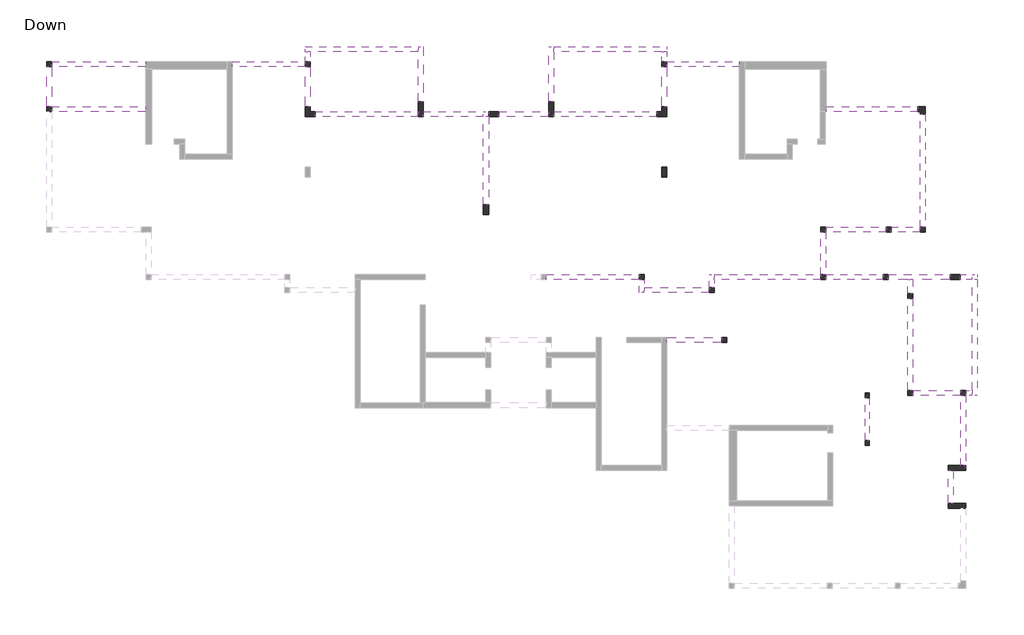
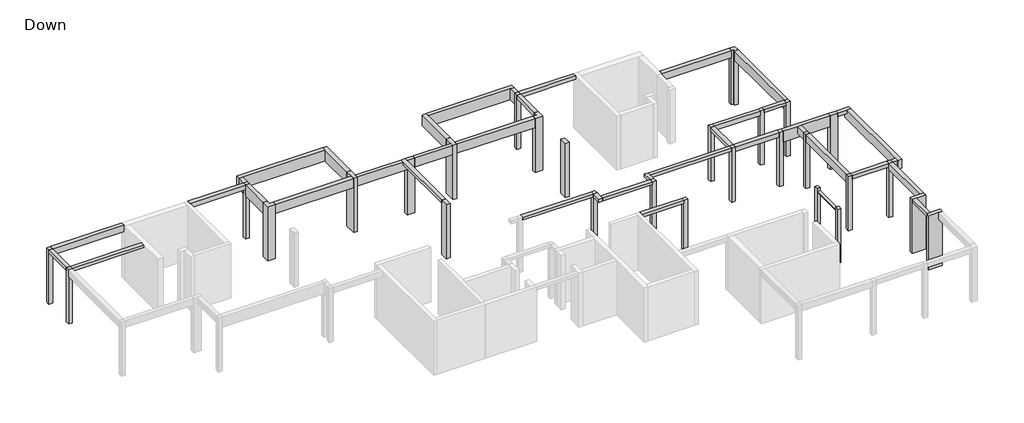
# One storey, part 2 of 2: 40 beams, 28 columns.
"""IFC4 building model written with IfcOpenShell, lengths in millimetres."""

from ifc_helpers import new_model, si_unit, frame, origin, origin_with_axes, place, context, project, spatial, polyline, outline, extrude, faceted_brep, element, save

model = new_model("IFC4")

# Units and contexts
model_context = context("Model", 3, world=origin())
ifc_project = project(units=[si_unit("LENGTHUNIT", "METRE", prefix="MILLI")], contexts=[model_context])

# Site, building, storey
site = spatial("IfcSite", under=ifc_project)
building = spatial("IfcBuilding", under=site)
storey = spatial("IfcBuildingStorey", under=building, Name="Down", Elevation=0.0)

# Beams
placement = place(None, origin())
element("IfcBeam", 1, ObjectType="Concrete Rectengular Beam : 16/20", at=placement, inside=storey, context=model_context, shape_type="SweptSolid", body=[
    extrude(outline(polyline([(36383.2842271, -26125.0806557), (36543.2842271, -26125.0806557), (36543.2842271, -27819.1243939), (36383.2842271, -27819.1243939), (36383.2842271, -26125.0806557)])), frame((0.0, 0.0, 2800.0), z_axis=(0.0, 0.0, 1.0), x_axis=(1.0, 0.0, 0.0)), (0.0, 0.0, 1.0), 40.0),
])
element("IfcBeam", 2, ObjectType="Concrete Rectengular Beam : 20/15", at=placement, inside=storey, context=model_context, shape_type="SweptSolid", body=[
    extrude(outline(polyline([(3764.5925114, -12916.1045626), (3964.5925114, -12916.1045626), (3964.5925114, -14517.2626845), (3764.5925114, -14517.2626845), (3764.5925114, -12916.1045626)])), frame((0.0, 0.0, 2850.0), z_axis=(0.0, 0.0, 1.0), x_axis=(1.0, 0.0, 0.0)), (0.0, 0.0, 1.0), 150.0),
])
element("IfcBeam", 3, ObjectType="Concrete Rectengular Beam : 20/15", at=placement, inside=storey, context=model_context, shape_type="SweptSolid", body=[
    extrude(outline(polyline([(3964.5925114, -14717.2626845), (3964.5925114, -14517.2626845), (7711.7769333, -14517.2626845), (7711.7769333, -14717.2626845), (3964.5925114, -14717.2626845)])), frame((0.0, 0.0, 2850.0), z_axis=(0.0, 0.0, 1.0), x_axis=(1.0, 0.0, 0.0)), (0.0, 0.0, 1.0), 150.0),
])
element("IfcBeam", 4, ObjectType="Concrete Rectengular Beam : 20/15", at=placement, inside=storey, context=model_context, shape_type="SweptSolid", body=[
    extrude(outline(polyline([(37421.6505657, -19524.5221497), (37421.6505657, -19324.5221497), (38580.9633489, -19324.5221497), (38580.9633489, -19524.5221497), (37421.6505657, -19524.5221497)])), frame((0.0, 0.0, 2850.0), z_axis=(0.0, 0.0, 1.0), x_axis=(1.0, 0.0, 0.0)), (0.0, 0.0, 1.0), 150.0),
])
element("IfcBeam", 5, ObjectType="Concrete Rectengular Beam : 20/15", at=placement, inside=storey, context=model_context, shape_type="SweptSolid", body=[
    extrude(outline(polyline([(39896.0050664, -30330.1793317), (39696.0050664, -30330.1793317), (39696.0050664, -29031.9248672), (39896.0050664, -29031.9248672), (39896.0050664, -30330.1793317)])), frame((0.0, 0.0, 2850.0), z_axis=(0.0, 0.0, 1.0), x_axis=(1.0, 0.0, 0.0)), (0.0, 0.0, 1.0), 150.0),
])
element("IfcBeam", 6, ObjectType="Concrete Rectengular Beam : 20/16", at=placement, inside=storey, context=model_context, shape_type="Brep", body=[
    faceted_brep([(21178.4466499, -18413.3840407, 3000.0), (21378.4466499, -18413.3840407, 3000.0), (21378.4466499, -14915.7476445, 3000.0), (21378.4466499, -14715.7476445, 3000.0), (21178.4466499, -14715.7476445, 3000.0), (21178.4466499, -14915.7476445, 3000.0), (21378.4466499, -18413.3840407, 2840.0), (21378.4466499, -14915.7476445, 2840.0), (21378.4466499, -14715.7476445, 2840.0), (21178.4466499, -18413.3840407, 2840.0), (21178.4466499, -14915.7476445, 2840.0), (21178.4466499, -14715.7476445, 2840.0)], [[[0, 1, 2, 3, 4, 5]], [[1, 6, 7, 8, 3, 2]], [[6, 9, 10, 11, 8, 7]], [[9, 0, 5, 4, 11, 10]], [[1, 0, 9, 6]], [[4, 3, 8, 11]]]),
])
element("IfcBeam", 7, ObjectType="Concrete Rectengular Beam : 20/16", at=placement, inside=storey, context=model_context, shape_type="SweptSolid", body=[
    extrude(outline(polyline([(27376.8445171, -21217.3313694), (27376.8445171, -21417.3313694), (23678.0627315, -21417.3313694), (23678.0627315, -21217.3313694), (27376.8445171, -21217.3313694)])), frame((0.0, 0.0, 2840.0), z_axis=(0.0, 0.0, 1.0), x_axis=(1.0, 0.0, 0.0)), (0.0, 0.0, 1.0), 160.0),
])
element("IfcBeam", 8, ObjectType="Concrete Rectengular Beam : 20/16", at=placement, inside=storey, context=model_context, shape_type="Brep", body=[
    faceted_brep([(27376.8445171, -21924.9991523, 3000.0), (27576.8445171, -21924.9991523, 3000.0), (27576.8445171, -21724.9991523, 3000.0), (27576.8445171, -21417.3313694, 3000.0), (27376.8445171, -21417.3313694, 3000.0), (27376.8445171, -21417.3313694, 2840.0), (27376.8445171, -21924.9991523, 2840.0), (27576.8445171, -21417.3313694, 2840.0), (27576.8445171, -21724.9991523, 2840.0), (27576.8445171, -21924.9991523, 2840.0)], [[[0, 1, 2, 3, 4]], [[4, 5, 6, 0]], [[5, 7, 8, 9, 6]], [[7, 3, 2, 1, 9, 8]], [[5, 4, 3, 7]], [[1, 0, 6, 9]]]),
])
element("IfcBeam", 9, ObjectType="Concrete Rectengular Beam : 20/16", at=placement, inside=storey, context=model_context, shape_type="SweptSolid", body=[
    extrude(outline(polyline([(30175.7089043, -21724.9991523), (30175.7089043, -21924.9991523), (27576.8445171, -21924.9991523), (27576.8445171, -21724.9991523), (30175.7089043, -21724.9991523)])), frame((0.0, 0.0, 2840.0), z_axis=(0.0, 0.0, 1.0), x_axis=(1.0, 0.0, 0.0)), (0.0, 0.0, 1.0), 160.0),
])
element("IfcBeam", 10, ObjectType="Concrete Rectengular Beam : 20/16", at=placement, inside=storey, context=model_context, shape_type="Brep", body=[
    faceted_brep([(30175.7089043, -21724.9991523, 3000.0), (30375.7089043, -21724.9991523, 3000.0), (30375.7089043, -21417.3313694, 3000.0), (30375.7089043, -21217.3313694, 3000.0), (30175.7089043, -21217.3313694, 3000.0), (30375.7089043, -21724.9991523, 2840.0), (30375.7089043, -21417.3313694, 2840.0), (30375.7089043, -21217.3313694, 2840.0), (30175.7089043, -21724.9991523, 2840.0), (30175.7089043, -21217.3313694, 2840.0)], [[[0, 1, 2, 3, 4]], [[1, 5, 6, 7, 3, 2]], [[5, 8, 9, 7, 6]], [[8, 0, 4, 9]], [[0, 8, 5, 1]], [[4, 3, 7, 9]]]),
])
element("IfcBeam", 11, ObjectType="Concrete Rectengular Beam : 20/16", at=placement, inside=storey, context=model_context, shape_type="SweptSolid", body=[
    extrude(outline(polyline([(34621.395755, -21217.3313694), (34621.395755, -21417.3313694), (30375.7089043, -21417.3313694), (30375.7089043, -21217.3313694), (34621.395755, -21217.3313694)])), frame((0.0, 0.0, 2840.0), z_axis=(0.0, 0.0, 1.0), x_axis=(1.0, 0.0, 0.0)), (0.0, 0.0, 1.0), 160.0),
])
element("IfcBeam", 12, ObjectType="Concrete Rectengular Beam : 20/16", at=placement, inside=storey, context=model_context, shape_type="SweptSolid", body=[
    extrude(outline(polyline([(30682.3560786, -23722.9713632), (30682.3560786, -23922.9713632), (28484.6380738, -23922.9713632), (28484.6380738, -23722.9713632), (30682.3560786, -23722.9713632)])), frame((0.0, 0.0, 2840.0), z_axis=(0.0, 0.0, 1.0), x_axis=(1.0, 0.0, 0.0)), (0.0, 0.0, 1.0), 160.0),
])
element("IfcBeam", 13, ObjectType="Concrete Rectengular Beam : 20/20", at=placement, inside=storey, context=model_context, shape_type="Brep", body=[
    faceted_brep([(28482.0540099, -12916.1045626, 3000.0), (28282.0540099, -12916.1045626, 3000.0), (28282.0540099, -14515.7476445, 3000.0), (28482.0540099, -14515.7476445, 3000.0), (28282.0540099, -12916.1045626, 2800.0), (28282.0540099, -14515.7476445, 2800.0), (28482.0540099, -12916.1045626, 2800.0), (28482.0540099, -14515.7476445, 2800.0), (28482.0540099, -14515.7476445, 2840.0), (28482.0540099, -12916.1045626, 2840.0)], [[[0, 1, 2, 3]], [[1, 4, 5, 2]], [[4, 6, 7, 5]], [[0, 3, 8, 7, 6, 9]], [[1, 0, 9, 6, 4]], [[3, 2, 5, 7, 8]]]),
])
element("IfcBeam", 14, ObjectType="Concrete Rectengular Beam : 20/20", at=placement, inside=storey, context=model_context, shape_type="Brep", body=[
    faceted_brep([(28482.0540099, -12716.1045626, 3000.0), (28482.0540099, -12916.1045626, 3000.0), (31380.8167217, -12916.1045626, 3000.0), (31380.8167217, -12716.1045626, 3000.0), (28482.0540099, -12916.1045626, 2840.0), (28482.0540099, -12916.1045626, 2800.0), (31380.8167217, -12916.1045626, 2800.0), (31380.8167217, -12916.1045626, 2840.0), (28482.0540099, -12716.1045626, 2800.0), (31380.8167217, -12716.1045626, 2800.0)], [[[0, 1, 2, 3]], [[1, 4, 5, 6, 7, 2]], [[5, 8, 9, 6]], [[8, 0, 3, 9]], [[0, 8, 5, 4, 1]], [[3, 2, 7, 6, 9]]]),
])
element("IfcBeam", 15, ObjectType="Concrete Rectengular Beam : 20/20", at=placement, inside=storey, context=model_context, shape_type="Brep", body=[
    faceted_brep([(34621.395755, -21217.3313694, 3000.0), (34821.395755, -21217.3313694, 3000.0), (34821.395755, -19524.5221497, 3000.0), (34621.395755, -19524.5221497, 3000.0), (34821.395755, -21217.3313694, 2800.0), (34821.395755, -19524.5221497, 2800.0), (34621.395755, -21217.3313694, 2800.0), (34621.395755, -19524.5221497, 2800.0), (34621.395755, -19524.5221497, 2840.0), (34621.395755, -21217.3313694, 2840.0)], [[[0, 1, 2, 3]], [[1, 4, 5, 2]], [[4, 6, 7, 5]], [[0, 3, 8, 7, 6, 9]], [[1, 0, 9, 6, 4]], [[3, 2, 5, 7, 8]]]),
])
element("IfcBeam", 16, ObjectType="Concrete Rectengular Beam : 20/20", at=placement, inside=storey, context=model_context, shape_type="Brep", body=[
    faceted_brep([(40184.8755666, -21217.3313694, 3000.0), (40184.8755666, -21417.3313694, 3000.0), (40664.8755666, -21417.3313694, 3000.0), (40864.8755666, -21417.3313694, 3000.0), (40864.8755666, -21217.3313694, 3000.0), (40184.8755666, -21417.3313694, 2800.0), (40664.8755666, -21417.3313694, 2800.0), (40864.8755666, -21417.3313694, 2800.0), (40184.8755666, -21217.3313694, 2800.0), (40664.8755666, -21217.3313694, 2800.0), (40864.8755666, -21217.3313694, 2800.0)], [[[0, 1, 2, 3, 4]], [[1, 5, 6, 7, 3, 2]], [[5, 8, 9, 10, 7, 6]], [[8, 0, 4, 10, 9]], [[1, 0, 8, 5]], [[4, 3, 7, 10]]]),
])
element("IfcBeam", 17, ObjectType="Concrete Rectengular Beam : 20/20", at=placement, inside=storey, context=model_context, shape_type="Brep", body=[
    faceted_brep([(40396.0050664, -25825.2456589, 3000.0), (40396.0050664, -26025.2456589, 3000.0), (40664.8755666, -26025.2456589, 3000.0), (40664.8755666, -25825.2456589, 3000.0), (40396.0050664, -26025.2456589, 2800.0), (40664.8755666, -26025.2456589, 2800.0), (40396.0050664, -25825.2456589, 2800.0), (40664.8755666, -25825.2456589, 2800.0), (40664.8755666, -25825.2456589, 2840.0)], [[[0, 1, 2, 3]], [[1, 4, 5, 2]], [[4, 6, 7, 5]], [[6, 0, 3, 8, 7]], [[1, 0, 6, 4]], [[3, 2, 5, 7, 8]]]),
])
element("IfcBeam", 18, ObjectType="Concrete Rectengular Beam : 20/20", at=placement, inside=storey, context=model_context, shape_type="Brep", body=[
    faceted_brep([(40196.0050664, -26025.2456589, 3000.0), (40196.0050664, -25825.2456589, 3000.0), (38283.1095165, -25825.2456589, 3000.0), (38283.1095165, -26025.2456589, 3000.0), (40196.0050664, -25825.2456589, 2800.0), (38283.1095165, -25825.2456589, 2800.0), (38283.1095165, -25825.2456589, 2840.0), (40196.0050664, -26025.2456589, 2800.0), (38283.1095165, -26025.2456589, 2800.0), (38283.1095165, -26025.2456589, 2840.0), (40196.0050664, -26025.2456589, 2840.0)], [[[0, 1, 2, 3]], [[1, 4, 5, 6, 2]], [[4, 7, 8, 5]], [[0, 3, 9, 8, 7, 10]], [[1, 0, 10, 7, 4]], [[3, 2, 6, 5, 8, 9]]]),
])
element("IfcBeam", 19, ObjectType="Concrete Rectengular Beam : 20/25", at=placement, inside=storey, context=model_context, shape_type="Brep", body=[
    faceted_brep([(14076.6245949, -12916.1045626, 3000.0), (14076.6245949, -12716.1045626, 3000.0), (11166.7769333, -12716.1045626, 3000.0), (11166.7769333, -12916.1045626, 3000.0), (14076.6245949, -12716.1045626, 2750.0), (11166.7769333, -12716.1045626, 2750.0), (14076.6245949, -12916.1045626, 2750.0), (11166.7769333, -12916.1045626, 2750.0), (14076.6245949, -12916.1045626, 2840.0), (11166.7769333, -12916.1045626, 2840.0)], [[[0, 1, 2, 3]], [[1, 4, 5, 2]], [[4, 6, 7, 5]], [[6, 8, 0, 3, 9, 7]], [[4, 1, 0, 8, 6]], [[3, 2, 5, 7, 9]]]),
])
element("IfcBeam", 20, ObjectType="Concrete Rectengular Beam : 20/25", at=placement, inside=storey, context=model_context, shape_type="Brep", body=[
    faceted_brep([(37118.3892225, -21417.3313694, 3000.0), (37118.3892225, -21217.3313694, 3000.0), (34821.395755, -21217.3313694, 3000.0), (34821.395755, -21417.3313694, 3000.0), (34821.395755, -21417.3313694, 2840.0), (34821.395755, -21417.3313694, 2750.0), (37118.3892225, -21417.3313694, 2750.0), (37118.3892225, -21417.3313694, 2840.0), (37118.3892225, -21217.3313694, 2750.0), (34821.395755, -21217.3313694, 2750.0)], [[[0, 1, 2, 3]], [[0, 3, 4, 5, 6, 7]], [[8, 6, 5, 9]], [[1, 8, 9, 2]], [[1, 0, 7, 6, 8]], [[3, 2, 9, 5, 4]]]),
])
element("IfcBeam", 21, ObjectType="Concrete Rectengular Beam : 20/25", at=placement, inside=storey, context=model_context, shape_type="Brep", body=[
    faceted_brep([(34821.395755, -19324.5221497, 3000.0), (34821.395755, -19524.5221497, 3000.0), (37221.6505657, -19524.5221497, 3000.0), (37221.6505657, -19324.5221497, 3000.0), (34821.395755, -19524.5221497, 2750.0), (37221.6505657, -19524.5221497, 2750.0), (34821.395755, -19324.5221497, 2750.0), (37221.6505657, -19324.5221497, 2750.0), (37221.6505657, -19324.5221497, 2840.0), (34821.395755, -19324.5221497, 2840.0)], [[[0, 1, 2, 3]], [[1, 4, 5, 2]], [[4, 6, 7, 5]], [[0, 3, 8, 7, 6, 9]], [[1, 0, 9, 6, 4]], [[3, 2, 5, 7, 8]]]),
])
element("IfcBeam", 22, ObjectType="Concrete Rectengular Beam : 20/35", at=placement, inside=storey, context=model_context, shape_type="Brep", body=[
    faceted_brep([(3964.5925114, -12716.1045626, 3000.0), (3964.5925114, -12916.1045626, 3000.0), (7711.7769333, -12916.1045626, 3000.0), (7711.7769333, -12716.1045626, 3000.0), (3964.5925114, -12916.1045626, 2840.0), (3964.5925114, -12916.1045626, 2650.0), (7711.7769333, -12916.1045626, 2650.0), (7711.7769333, -12916.1045626, 2840.0), (3964.5925114, -12716.1045626, 2650.0), (7711.7769333, -12716.1045626, 2650.0)], [[[0, 1, 2, 3]], [[1, 4, 5, 6, 7, 2]], [[5, 8, 9, 6]], [[8, 0, 3, 9]], [[1, 0, 8, 5, 4]], [[3, 2, 7, 6, 9]]]),
])
element("IfcBeam", 23, ObjectType="Concrete Rectengular Beam : 20/35", at=placement, inside=storey, context=model_context, shape_type="Brep", body=[
    faceted_brep([(40394.7023527, -28931.9248672, 3000.0), (40396.0050664, -28931.9248672, 3000.0), (40396.0050664, -26025.2456589, 3000.0), (40196.0050664, -26025.2456589, 3000.0), (40196.0050664, -28831.9248672, 3000.0), (40394.7023527, -28831.9248672, 3000.0), (40196.0050664, -28831.9248672, 2650.0), (40196.0050664, -28831.9248672, 2840.0), (40196.0050664, -26025.2456589, 2840.0), (40196.0050664, -26025.2456589, 2650.0), (40396.0050664, -28931.9248672, 2650.0), (40394.7023527, -28931.9248672, 2650.0), (40394.7023527, -28831.9248672, 2650.0), (40396.0050664, -26025.2456589, 2650.0)], [[[0, 1, 2, 3, 4, 5]], [[6, 7, 4, 3, 8, 9]], [[10, 11, 12, 6, 9, 13]], [[1, 10, 13, 2]], [[10, 1, 0, 11]], [[12, 5, 4, 7, 6]], [[5, 12, 11, 0]], [[3, 2, 13, 9, 8]]]),
])
element("IfcBeam", 24, ObjectType="Concrete Rectengular Beam : 20/40", at=placement, inside=storey, context=model_context, shape_type="Brep", body=[
    faceted_brep([(38083.1095165, -21967.4922699, 3000.0), (38283.1095165, -21967.4922699, 3000.0), (38283.1095165, -21417.3313694, 3000.0), (38083.1095165, -21417.3313694, 3000.0), (38283.1095165, -21967.4922699, 2600.0), (38283.1095165, -21417.3313694, 2600.0), (38283.1095165, -21417.3313694, 2840.0), (38083.1095165, -21967.4922699, 2600.0), (38083.1095165, -21417.3313694, 2600.0), (38083.1095165, -21417.3313694, 2840.0), (38083.1095165, -21967.4922699, 2840.0)], [[[0, 1, 2, 3]], [[1, 4, 5, 6, 2]], [[4, 7, 8, 5]], [[0, 3, 9, 8, 7, 10]], [[1, 0, 10, 7, 4]], [[3, 2, 6, 5, 8, 9]]]),
])
element("IfcBeam", 25, ObjectType="Concrete Rectengular Beam : 20/40", at=placement, inside=storey, context=model_context, shape_type="Brep", body=[
    faceted_brep([(38083.1095165, -25825.2456589, 3000.0), (38283.1095165, -25825.2456589, 3000.0), (38283.1095165, -22167.4922699, 3000.0), (38083.1095165, -22167.4922699, 3000.0), (38083.1095165, -22167.4922699, 2840.0), (38083.1095165, -22167.4922699, 2600.0), (38083.1095165, -25825.2456589, 2600.0), (38083.1095165, -25825.2456589, 2840.0), (38283.1095165, -25825.2456589, 2600.0), (38283.1095165, -22167.4922699, 2600.0), (38283.1095165, -25825.2456589, 2840.0)], [[[0, 1, 2, 3]], [[0, 3, 4, 5, 6, 7]], [[8, 6, 5, 9]], [[1, 10, 8, 9, 2]], [[1, 0, 7, 6, 8, 10]], [[3, 2, 9, 5, 4]]]),
])
element("IfcBeam", 26, ObjectType="Concrete Rectengular Beam : 20/40", at=placement, inside=storey, context=model_context, shape_type="Brep", body=[
    faceted_brep([(38480.9633489, -14717.2626845, 3000.0), (38480.9633489, -14517.2626845, 3000.0), (34840.8167217, -14517.2626845, 3000.0), (34840.8167217, -14717.2626845, 3000.0), (38480.9633489, -14517.2626845, 2600.0), (34840.8167217, -14517.2626845, 2600.0), (38480.9633489, -14717.2626845, 2600.0), (34840.8167217, -14717.2626845, 2600.0), (34840.8167217, -14717.2626845, 2840.0), (38480.9633489, -14717.2626845, 2840.0)], [[[0, 1, 2, 3]], [[1, 4, 5, 2]], [[4, 6, 7, 5]], [[0, 3, 8, 7, 6, 9]], [[1, 0, 9, 6, 4]], [[3, 2, 5, 7, 8]]]),
])
element("IfcBeam", 27, ObjectType="Concrete Rectengular Beam : 20/50", at=placement, inside=storey, context=model_context, shape_type="Brep", body=[
    faceted_brep([(23784.4934221, -14915.7476445, 3000.0), (23784.4934221, -14715.7476445, 3000.0), (21780.7780067, -14715.7476445, 3000.0), (21780.7780067, -14915.7476445, 3000.0), (21780.7780067, -14915.7476445, 2840.0), (21780.7780067, -14915.7476445, 2500.0), (23784.4934221, -14915.7476445, 2500.0), (23784.4934221, -14915.7476445, 2840.0), (23784.4934221, -14715.7476445, 2500.0), (21780.7780067, -14715.7476445, 2500.0)], [[[0, 1, 2, 3]], [[0, 3, 4, 5, 6, 7]], [[8, 6, 5, 9]], [[1, 8, 9, 2]], [[1, 0, 7, 6, 8]], [[3, 2, 9, 5, 4]]]),
])
element("IfcBeam", 28, ObjectType="Concrete Rectengular Beam : 20/50", at=placement, inside=storey, context=model_context, shape_type="Brep", body=[
    faceted_brep([(23984.4934221, -14715.7476445, 3000.0), (23984.4934221, -14915.7476445, 3000.0), (28082.0540099, -14915.7476445, 3000.0), (28082.0540099, -14715.7476445, 3000.0), (23984.4934221, -14915.7476445, 2840.0), (23984.4934221, -14915.7476445, 2500.0), (28082.0540099, -14915.7476445, 2500.0), (28082.0540099, -14915.7476445, 2840.0), (23984.4934221, -14715.7476445, 2500.0), (28082.0540099, -14715.7476445, 2500.0), (23984.4934221, -14715.7476445, 2840.0)], [[[0, 1, 2, 3]], [[2, 1, 4, 5, 6, 7]], [[5, 8, 9, 6]], [[8, 10, 0, 3, 9]], [[1, 0, 10, 8, 5, 4]], [[3, 2, 7, 6, 9]]]),
])
element("IfcBeam", 29, ObjectType="Concrete Rectengular Beam : 20/50", at=placement, inside=storey, context=model_context, shape_type="Brep", body=[
    faceted_brep([(18776.6245949, -14715.7476445, 3000.0), (18776.6245949, -14915.7476445, 3000.0), (21178.4466499, -14915.7476445, 3000.0), (21178.4466499, -14715.7476445, 3000.0), (21378.4466499, -14715.7476445, 2500.0), (18776.6245949, -14715.7476445, 2500.0), (21178.4466499, -14715.7476445, 2840.0), (21378.4466499, -14715.7476445, 2840.0), (21378.4466499, -14915.7476445, 2500.0), (18776.6245949, -14915.7476445, 2500.0), (21378.4466499, -14915.7476445, 2840.0), (21178.4466499, -14915.7476445, 2840.0), (18776.6245949, -14915.7476445, 2840.0)], [[[0, 1, 2, 3]], [[4, 5, 0, 3, 6, 7]], [[4, 8, 9, 5]], [[9, 8, 10, 11, 2, 1, 12]], [[8, 4, 7, 10]], [[1, 0, 5, 9, 12]], [[6, 11, 10, 7]], [[11, 6, 3, 2]]]),
])
element("IfcBeam", 30, ObjectType="Concrete Rectengular Beam : 20/50", at=placement, inside=storey, context=model_context, shape_type="Brep", body=[
    faceted_brep([(18576.6245949, -14915.7476445, 3000.0), (18576.6245949, -14715.7476445, 3000.0), (14476.6245949, -14715.7476445, 3000.0), (14476.6245949, -14915.7476445, 3000.0), (18576.6245949, -14715.7476445, 2840.0), (18576.6245949, -14715.7476445, 2500.0), (14476.6245949, -14715.7476445, 2500.0), (18576.6245949, -14915.7476445, 2500.0), (14476.6245949, -14915.7476445, 2500.0), (14476.6245949, -14915.7476445, 2840.0), (18576.6245949, -14915.7476445, 2840.0)], [[[0, 1, 2, 3]], [[1, 4, 5, 6, 2]], [[5, 7, 8, 6]], [[0, 3, 9, 8, 7, 10]], [[1, 0, 10, 7, 5, 4]], [[3, 2, 6, 8, 9]]]),
])
element("IfcBeam", 31, ObjectType="Concrete Rectengular Beam : 20/50", at=placement, inside=storey, context=model_context, shape_type="Brep", body=[
    faceted_brep([(40664.8755666, -26025.2456589, 3000.0), (40864.8755666, -26025.2456589, 3000.0), (40864.8755666, -21417.3313694, 3000.0), (40664.8755666, -21417.3313694, 3000.0), (40664.8755666, -25825.2456589, 3000.0), (40664.8755666, -21217.3313694, 2500.0), (40664.8755666, -26025.2456589, 2500.0), (40664.8755666, -26025.2456589, 2800.0), (40664.8755666, -21417.3313694, 2840.0), (40664.8755666, -21417.3313694, 2800.0), (40664.8755666, -21217.3313694, 2800.0), (40864.8755666, -21217.3313694, 2500.0), (40864.8755666, -26025.2456589, 2500.0), (40864.8755666, -21217.3313694, 2800.0), (40864.8755666, -21417.3313694, 2800.0)], [[[0, 1, 2, 3, 4]], [[5, 6, 7, 0, 4, 3, 8, 9, 10]], [[5, 11, 12, 6]], [[12, 11, 13, 14, 2, 1]], [[11, 5, 10, 13]], [[1, 0, 7, 6, 12]], [[14, 9, 8, 3, 2]], [[9, 14, 13, 10]]]),
])
element("IfcBeam", 32, ObjectType="Concrete Rectengular Beam : 20/50", at=placement, inside=storey, context=model_context, shape_type="Brep", body=[
    faceted_brep([(38580.9633489, -19324.5221497, 3000.0), (38780.9633489, -19324.5221497, 3000.0), (38780.9633489, -14817.2626845, 3000.0), (38580.9633489, -14817.2626845, 3000.0), (38780.9633489, -19324.5221497, 2500.0), (38780.9633489, -14817.2626845, 2500.0), (38580.9633489, -19324.5221497, 2500.0), (38580.9633489, -14817.2626845, 2500.0), (38580.9633489, -19324.5221497, 2840.0)], [[[0, 1, 2, 3]], [[1, 4, 5, 2]], [[4, 6, 7, 5]], [[6, 8, 0, 3, 7]], [[1, 0, 8, 6, 4]], [[3, 2, 5, 7]]]),
])
element("IfcBeam", 33, ObjectType="Concrete Rectengular Beam : 20/60", at=placement, inside=storey, context=model_context, shape_type="Brep", body=[
    faceted_brep([(23784.4934221, -14317.2626845, 3000.0), (23984.4934221, -14317.2626845, 3000.0), (23984.4934221, -12317.2626845, 3000.0), (23984.4934221, -12117.2626845, 3000.0), (23784.4934221, -12117.2626845, 3000.0), (23984.4934221, -14317.2626845, 2400.0), (23984.4934221, -12317.2626845, 2400.0), (23984.4934221, -12117.2626845, 2400.0), (23784.4934221, -14317.2626845, 2400.0), (23784.4934221, -12117.2626845, 2400.0)], [[[0, 1, 2, 3, 4]], [[1, 5, 6, 7, 3, 2]], [[5, 8, 9, 7, 6]], [[8, 0, 4, 9]], [[1, 0, 8, 5]], [[4, 3, 7, 9]]]),
])
element("IfcBeam", 34, ObjectType="Concrete Rectengular Beam : 20/60", at=placement, inside=storey, context=model_context, shape_type="Brep", body=[
    faceted_brep([(28482.0540099, -12317.2626845, 3000.0), (28482.0540099, -12117.2626845, 3000.0), (23984.4934221, -12117.2626845, 3000.0), (23984.4934221, -12317.2626845, 3000.0), (28282.0540099, -12317.2626845, 3000.0), (28482.0540099, -12317.2626845, 2400.0), (23984.4934221, -12317.2626845, 2840.0), (23984.4934221, -12317.2626845, 2400.0), (28282.0540099, -12317.2626845, 2400.0), (28482.0540099, -12117.2626845, 2400.0), (23984.4934221, -12117.2626845, 2400.0)], [[[0, 1, 2, 3, 4]], [[5, 0, 4, 3, 6, 7, 8]], [[9, 5, 8, 7, 10]], [[1, 9, 10, 2]], [[3, 2, 10, 7, 6]], [[1, 0, 5, 9]]]),
])
element("IfcBeam", 35, ObjectType="Concrete Rectengular Beam : 20/60", at=placement, inside=storey, context=model_context, shape_type="Brep", body=[
    faceted_brep([(28282.0540099, -12716.1045626, 3000.0), (28482.0540099, -12716.1045626, 3000.0), (28482.0540099, -12317.2626845, 3000.0), (28282.0540099, -12317.2626845, 3000.0), (28282.0540099, -12716.1045626, 2400.0), (28282.0540099, -12317.2626845, 2840.0), (28282.0540099, -12317.2626845, 2400.0), (28482.0540099, -12716.1045626, 2400.0), (28482.0540099, -12317.2626845, 2400.0)], [[[0, 1, 2, 3]], [[4, 0, 3, 5, 6]], [[7, 4, 6, 8]], [[1, 7, 8, 2]], [[1, 0, 4, 7]], [[3, 2, 8, 6, 5]]]),
])
element("IfcBeam", 36, ObjectType="Concrete Rectengular Beam : 20/60", at=placement, inside=storey, context=model_context, shape_type="Brep", body=[
    faceted_brep([(18576.6245949, -14317.2626845, 3000.0), (18776.6245949, -14317.2626845, 3000.0), (18776.6245949, -12117.2626845, 3000.0), (18576.6245949, -12117.2626845, 3000.0), (18576.6245949, -12317.2626845, 3000.0), (18776.6245949, -14317.2626845, 2400.0), (18776.6245949, -12117.2626845, 2400.0), (18576.6245949, -14317.2626845, 2400.0), (18576.6245949, -12317.2626845, 2400.0), (18576.6245949, -12117.2626845, 2400.0)], [[[0, 1, 2, 3, 4]], [[1, 5, 6, 2]], [[5, 7, 8, 9, 6]], [[7, 0, 4, 3, 9, 8]], [[1, 0, 7, 5]], [[3, 2, 6, 9]]]),
])
element("IfcBeam", 37, ObjectType="Concrete Rectengular Beam : 20/60", at=placement, inside=storey, context=model_context, shape_type="Brep", body=[
    faceted_brep([(14076.6245949, -12117.2626845, 3000.0), (14076.6245949, -12317.2626845, 3000.0), (14276.6245949, -12317.2626845, 3000.0), (18576.6245949, -12317.2626845, 3000.0), (18576.6245949, -12117.2626845, 3000.0), (14076.6245949, -12117.2626845, 2400.0), (18576.6245949, -12117.2626845, 2400.0), (14076.6245949, -12317.2626845, 2400.0), (18576.6245949, -12317.2626845, 2400.0), (14276.6245949, -12317.2626845, 2400.0), (18576.6245949, -12317.2626845, 2840.0)], [[[0, 1, 2, 3, 4]], [[5, 0, 4, 6]], [[7, 5, 6, 8, 9]], [[1, 7, 9, 8, 10, 3, 2]], [[4, 3, 10, 8, 6]], [[1, 0, 5, 7]]]),
])
element("IfcBeam", 38, ObjectType="Concrete Rectengular Beam : 20/60", at=placement, inside=storey, context=model_context, shape_type="Brep", body=[
    faceted_brep([(14276.6245949, -12317.2626845, 3000.0), (14076.6245949, -12317.2626845, 3000.0), (14076.6245949, -12716.1045626, 3000.0), (14276.6245949, -12716.1045626, 3000.0), (14076.6245949, -12317.2626845, 2400.0), (14076.6245949, -12716.1045626, 2400.0), (14276.6245949, -12317.2626845, 2400.0), (14276.6245949, -12716.1045626, 2400.0), (14276.6245949, -12317.2626845, 2840.0)], [[[0, 1, 2, 3]], [[1, 4, 5, 2]], [[4, 6, 7, 5]], [[6, 8, 0, 3, 7]], [[1, 0, 8, 6, 4]], [[3, 2, 5, 7]]]),
])
element("IfcBeam", 39, ObjectType="Concrete Rectengular Beam : 20/60", at=placement, inside=storey, context=model_context, shape_type="Brep", body=[
    faceted_brep([(14276.6245949, -12916.1045626, 3000.0), (14076.6245949, -12916.1045626, 3000.0), (14076.6245949, -14515.7476445, 3000.0), (14276.6245949, -14515.7476445, 3000.0), (14076.6245949, -12916.1045626, 2840.0), (14076.6245949, -12916.1045626, 2400.0), (14076.6245949, -14515.7476445, 2400.0), (14076.6245949, -14515.7476445, 2840.0), (14276.6245949, -12916.1045626, 2400.0), (14276.6245949, -14515.7476445, 2400.0)], [[[0, 1, 2, 3]], [[2, 1, 4, 5, 6, 7]], [[5, 8, 9, 6]], [[8, 0, 3, 9]], [[1, 0, 8, 5, 4]], [[3, 2, 7, 6, 9]]]),
])
element("IfcBeam", 40, ObjectType="Concrete Rectengular Beam : 20/60", at=placement, inside=storey, context=model_context, shape_type="Brep", body=[
    faceted_brep([(37318.3892225, -21217.3313694, 3000.0), (37318.3892225, -21417.3313694, 3000.0), (38083.1095165, -21417.3313694, 3000.0), (38283.1095165, -21417.3313694, 3000.0), (39784.8755666, -21417.3313694, 3000.0), (39784.8755666, -21217.3313694, 3000.0), (37318.3892225, -21417.3313694, 2400.0), (39784.8755666, -21417.3313694, 2400.0), (37318.3892225, -21417.3313694, 2840.0), (37318.3892225, -21217.3313694, 2400.0), (39784.8755666, -21217.3313694, 2400.0)], [[[0, 1, 2, 3, 4, 5]], [[6, 7, 4, 3, 2, 1, 8]], [[6, 9, 10, 7]], [[9, 0, 5, 10]], [[1, 0, 9, 6, 8]], [[5, 4, 7, 10]]]),
])

# Columns
element("IfcColumn", 41, ObjectType="Concrete Rectengular Column : 16/20", at=placement, inside=storey, context=model_context, shape_type="Brep", body=[
    faceted_brep([(36543.2842271, -25925.0806557, 0.0), (36543.2842271, -26125.0806557, 0.0), (36383.2842271, -26125.0806557, 0.0), (36383.2842271, -25925.0806557, 0.0), (36543.2842271, -25925.0806557, 3000.0), (36543.2842271, -26125.0806557, 3000.0), (36543.2842271, -26125.0806557, 2840.0), (36543.2842271, -25925.0806557, 2840.0), (36383.2842271, -26125.0806557, 3000.0), (36383.2842271, -26125.0806557, 2840.0), (36383.2842271, -25925.0806557, 3000.0), (36383.2842271, -25925.0806557, 2840.0)], [[[0, 1, 2, 3]], [[4, 5, 6, 1, 0, 7]], [[5, 8, 9, 2, 1, 6]], [[8, 10, 11, 3, 2, 9]], [[10, 4, 7, 0, 3, 11]], [[4, 10, 8, 5]]]),
])
element("IfcColumn", 42, ObjectType="Concrete Rectengular Column : 16/20", at=placement, inside=storey, context=model_context, shape_type="Brep", body=[
    faceted_brep([(36543.2842271, -27819.1243939, 0.0), (36543.2842271, -28019.1243939, 0.0), (36383.2842271, -28019.1243939, 0.0), (36383.2842271, -27819.1243939, 0.0), (36543.2842271, -27819.1243939, 3000.0), (36543.2842271, -28019.1243939, 3000.0), (36543.2842271, -28019.1243939, 2840.0), (36543.2842271, -27819.1243939, 2840.0), (36383.2842271, -28019.1243939, 3000.0), (36383.2842271, -28019.1243939, 2840.0), (36383.2842271, -27819.1243939, 3000.0), (36383.2842271, -27819.1243939, 2840.0)], [[[0, 1, 2, 3]], [[4, 5, 6, 1, 0, 7]], [[5, 8, 9, 2, 1, 6]], [[8, 10, 11, 3, 2, 9]], [[10, 4, 7, 0, 3, 11]], [[4, 10, 8, 5]]]),
])
element("IfcColumn", 43, ObjectType="Concrete Rectengular Column : 20/20", at=placement, inside=storey, context=model_context, shape_type="SweptSolid", body=[
    extrude(outline(polyline([(40396.0050664, -25825.2456589), (40396.0050664, -26025.2456589), (40196.0050664, -26025.2456589), (40196.0050664, -25825.2456589), (40396.0050664, -25825.2456589)])), origin_with_axes(), (0.0, 0.0, 1.0), 3000.0),
])
element("IfcColumn", 44, ObjectType="Concrete Rectengular Column : 20/20", at=placement, inside=storey, context=model_context, shape_type="Brep", body=[
    faceted_brep([(38283.1095165, -25825.2456589, 0.0), (38283.1095165, -26025.2456589, 0.0), (38083.1095165, -26025.2456589, 0.0), (38083.1095165, -25825.2456589, 0.0), (38283.1095165, -25825.2456589, 3000.0), (38283.1095165, -26025.2456589, 3000.0), (38083.1095165, -26025.2456589, 3000.0), (38083.1095165, -26025.2456589, 2840.0), (38083.1095165, -25825.2456589, 3000.0)], [[[0, 1, 2, 3]], [[4, 5, 1, 0]], [[5, 6, 7, 2, 1]], [[6, 8, 3, 2, 7]], [[8, 4, 0, 3]], [[4, 8, 6, 5]]]),
])
element("IfcColumn", 45, ObjectType="Concrete Rectengular Column : 20/20", at=placement, inside=storey, context=model_context, shape_type="SweptSolid", body=[
    extrude(outline(polyline([(38283.1095165, -21967.4922699), (38283.1095165, -22167.4922699), (38083.1095165, -22167.4922699), (38083.1095165, -21967.4922699), (38283.1095165, -21967.4922699)])), origin_with_axes(), (0.0, 0.0, 1.0), 3000.0),
])
element("IfcColumn", 46, ObjectType="Concrete Rectengular Column : 20/20", at=placement, inside=storey, context=model_context, shape_type="SweptSolid", body=[
    extrude(outline(polyline([(37318.3892225, -21217.3313694), (37318.3892225, -21417.3313694), (37118.3892225, -21417.3313694), (37118.3892225, -21217.3313694), (37318.3892225, -21217.3313694)])), origin_with_axes(), (0.0, 0.0, 1.0), 3000.0),
])
element("IfcColumn", 47, ObjectType="Concrete Rectengular Column : 20/20", at=placement, inside=storey, context=model_context, shape_type="SweptSolid", body=[
    extrude(outline(polyline([(34821.395755, -21217.3313694), (34821.395755, -21417.3313694), (34621.395755, -21417.3313694), (34621.395755, -21217.3313694), (34821.395755, -21217.3313694)])), origin_with_axes(), (0.0, 0.0, 1.0), 3000.0),
])
element("IfcColumn", 48, ObjectType="Concrete Rectengular Column : 20/20", at=placement, inside=storey, context=model_context, shape_type="Brep", body=[
    faceted_brep([(30375.7089043, -21724.9991523, 0.0), (30375.7089043, -21924.9991523, 0.0), (30175.7089043, -21924.9991523, 0.0), (30175.7089043, -21724.9991523, 0.0), (30375.7089043, -21724.9991523, 3000.0), (30375.7089043, -21924.9991523, 3000.0), (30375.7089043, -21924.9991523, 2840.0), (30175.7089043, -21924.9991523, 3000.0), (30175.7089043, -21724.9991523, 3000.0)], [[[0, 1, 2, 3]], [[4, 5, 6, 1, 0]], [[5, 7, 2, 1, 6]], [[7, 8, 3, 2]], [[8, 4, 0, 3]], [[4, 8, 7, 5]]]),
])
element("IfcColumn", 49, ObjectType="Concrete Rectengular Column : 20/20", at=placement, inside=storey, context=model_context, shape_type="Brep", body=[
    faceted_brep([(27576.8445171, -21217.3313694, 0.0), (27576.8445171, -21417.3313694, 0.0), (27376.8445171, -21417.3313694, 0.0), (27376.8445171, -21217.3313694, 0.0), (27576.8445171, -21217.3313694, 3000.0), (27576.8445171, -21417.3313694, 3000.0), (27576.8445171, -21217.3313694, 2840.0), (27376.8445171, -21417.3313694, 3000.0), (27376.8445171, -21217.3313694, 3000.0)], [[[0, 1, 2, 3]], [[4, 5, 1, 0, 6]], [[5, 7, 2, 1]], [[7, 8, 3, 2]], [[8, 4, 6, 0, 3]], [[4, 8, 7, 5]]]),
])
element("IfcColumn", 50, ObjectType="Concrete Rectengular Column : 20/20", at=placement, inside=storey, context=model_context, shape_type="Brep", body=[
    faceted_brep([(30882.3560786, -23722.9713632, 0.0), (30882.3560786, -23922.9713632, 0.0), (30682.3560786, -23922.9713632, 0.0), (30682.3560786, -23722.9713632, 0.0), (30882.3560786, -23722.9713632, 3000.0), (30882.3560786, -23922.9713632, 3000.0), (30882.3560786, -23922.9713632, 2840.0), (30882.3560786, -23722.9713632, 2840.0), (30682.3560786, -23922.9713632, 3000.0), (30682.3560786, -23722.9713632, 3000.0)], [[[0, 1, 2, 3]], [[4, 5, 6, 1, 0, 7]], [[5, 8, 2, 1, 6]], [[8, 9, 3, 2]], [[9, 4, 7, 0, 3]], [[4, 9, 8, 5]]]),
])
element("IfcColumn", 51, ObjectType="Concrete Rectengular Column : 20/20", at=placement, inside=storey, context=model_context, shape_type="Brep", body=[
    faceted_brep([(34821.395755, -19324.5221497, 0.0), (34821.395755, -19524.5221497, 0.0), (34621.395755, -19524.5221497, 0.0), (34621.395755, -19324.5221497, 0.0), (34821.395755, -19324.5221497, 3000.0), (34821.395755, -19524.5221497, 3000.0), (34621.395755, -19524.5221497, 3000.0), (34621.395755, -19324.5221497, 3000.0), (34621.395755, -19324.5221497, 2840.0)], [[[0, 1, 2, 3]], [[4, 5, 1, 0]], [[5, 6, 2, 1]], [[6, 7, 8, 3, 2]], [[7, 4, 0, 3, 8]], [[4, 7, 6, 5]]]),
])
element("IfcColumn", 52, ObjectType="Concrete Rectengular Column : 20/20", at=placement, inside=storey, context=model_context, shape_type="SweptSolid", body=[
    extrude(outline(polyline([(37421.6505657, -19324.5221497), (37421.6505657, -19524.5221497), (37221.6505657, -19524.5221497), (37221.6505657, -19324.5221497), (37421.6505657, -19324.5221497)])), origin_with_axes(), (0.0, 0.0, 1.0), 3000.0),
])
element("IfcColumn", 53, ObjectType="Concrete Rectengular Column : 20/20", at=placement, inside=storey, context=model_context, shape_type="SweptSolid", body=[
    extrude(outline(polyline([(38780.9633489, -19324.5221497), (38780.9633489, -19524.5221497), (38580.9633489, -19524.5221497), (38580.9633489, -19324.5221497), (38780.9633489, -19324.5221497)])), origin_with_axes(), (0.0, 0.0, 1.0), 3000.0),
])
element("IfcColumn", 54, ObjectType="Concrete Rectengular Column : 20/20", at=placement, inside=storey, context=model_context, shape_type="SweptSolid", body=[
    extrude(outline(polyline([(28482.0540099, -12716.1045626), (28482.0540099, -12916.1045626), (28282.0540099, -12916.1045626), (28282.0540099, -12716.1045626), (28482.0540099, -12716.1045626)])), origin_with_axes(), (0.0, 0.0, 1.0), 3000.0),
])
element("IfcColumn", 55, ObjectType="Concrete Rectengular Column : 20/20", at=placement, inside=storey, context=model_context, shape_type="Brep", body=[
    faceted_brep([(14276.6245949, -12716.1045626, 0.0), (14276.6245949, -12916.1045626, 0.0), (14076.6245949, -12916.1045626, 0.0), (14076.6245949, -12716.1045626, 0.0), (14276.6245949, -12716.1045626, 3000.0), (14276.6245949, -12916.1045626, 3000.0), (14276.6245949, -12916.1045626, 2400.0), (14276.6245949, -12716.1045626, 2400.0), (14076.6245949, -12916.1045626, 3000.0), (14076.6245949, -12916.1045626, 2400.0), (14076.6245949, -12716.1045626, 3000.0), (14076.6245949, -12716.1045626, 2400.0)], [[[0, 1, 2, 3]], [[4, 5, 6, 1, 0, 7]], [[5, 8, 9, 2, 1, 6]], [[8, 10, 11, 3, 2, 9]], [[10, 4, 7, 0, 3, 11]], [[4, 10, 8, 5]]]),
])
element("IfcColumn", 56, ObjectType="Concrete Rectengular Column : 20/20", at=placement, inside=storey, context=model_context, shape_type="SweptSolid", body=[
    extrude(outline(polyline([(3964.5925114, -12716.1045626), (3964.5925114, -12916.1045626), (3764.5925114, -12916.1045626), (3764.5925114, -12716.1045626), (3964.5925114, -12716.1045626)])), origin_with_axes(), (0.0, 0.0, 1.0), 3000.0),
])
element("IfcColumn", 57, ObjectType="Concrete Rectengular Column : 20/20", at=placement, inside=storey, context=model_context, shape_type="SweptSolid", body=[
    extrude(outline(polyline([(3964.5925114, -14517.2626845), (3964.5925114, -14717.2626845), (3764.5925114, -14717.2626845), (3764.5925114, -14517.2626845), (3964.5925114, -14517.2626845)])), origin_with_axes(), (0.0, 0.0, 1.0), 3000.0),
])
element("IfcColumn", 58, ObjectType="Concrete Rectengular Column : 20/40", at=placement, inside=storey, context=model_context, shape_type="SweptSolid", body=[
    extrude(outline(polyline([(39784.8755666, -21217.3313694), (40184.8755666, -21217.3313694), (40184.8755666, -21417.3313694), (39784.8755666, -21417.3313694), (39784.8755666, -21217.3313694)])), origin_with_axes(), (0.0, 0.0, 1.0), 3000.0),
])
element("IfcColumn", 59, ObjectType="Concrete Rectengular Column : 20/40", at=placement, inside=storey, context=model_context, shape_type="SweptSolid", body=[
    extrude(outline(polyline([(21380.7780067, -14715.7476445), (21780.7780067, -14715.7476445), (21780.7780067, -14915.7476445), (21380.7780067, -14915.7476445), (21380.7780067, -14715.7476445)])), origin_with_axes(), (0.0, 0.0, 1.0), 3000.0),
])
element("IfcColumn", 60, ObjectType="Concrete Rectengular Column : 20/40", at=placement, inside=storey, context=model_context, shape_type="Brep", body=[
    faceted_brep([(21378.4466499, -18413.3840407, 0.0), (21378.4466499, -18813.3840407, 0.0), (21178.4466499, -18813.3840407, 0.0), (21178.4466499, -18413.3840407, 0.0), (21378.4466499, -18413.3840407, 3000.0), (21378.4466499, -18813.3840407, 3000.0), (21378.4466499, -18813.3840407, 2840.0), (21178.4466499, -18813.3840407, 3000.0), (21178.4466499, -18813.3840407, 2840.0), (21178.4466499, -18413.3840407, 3000.0)], [[[0, 1, 2, 3]], [[4, 5, 6, 1, 0]], [[5, 7, 8, 2, 1, 6]], [[7, 9, 3, 2, 8]], [[9, 4, 0, 3]], [[4, 9, 7, 5]]]),
])
element("IfcColumn", 61, ObjectType="Concrete Rectengular Column : 20/40", at=placement, inside=storey, context=model_context, shape_type="Brep", body=[
    faceted_brep([(28476.6245949, -16922.7697624, 0.0), (28476.6245949, -17322.7697624, 0.0), (28276.6245949, -17322.7697624, 0.0), (28276.6245949, -16922.7697624, 0.0), (28476.6245949, -16922.7697624, 3000.0), (28476.6245949, -17322.7697624, 3000.0), (28476.6245949, -17322.7697624, 2840.0), (28476.6245949, -16922.7697624, 2840.0), (28276.6245949, -17322.7697624, 3000.0), (28276.6245949, -17322.7697624, 2840.0), (28276.6245949, -16922.7697624, 3000.0), (28276.6245949, -16922.7697624, 2840.0)], [[[0, 1, 2, 3]], [[4, 5, 6, 1, 0, 7]], [[5, 8, 9, 2, 1, 6]], [[8, 10, 11, 3, 2, 9]], [[10, 4, 7, 0, 3, 11]], [[4, 10, 8, 5]]]),
])
element("IfcColumn", 62, ObjectType="Concrete Rectengular Column : 20/60", at=placement, inside=storey, context=model_context, shape_type="Brep", body=[
    faceted_brep([(23984.4934221, -14317.2626845, 0.0), (23984.4934221, -14917.2626845, 0.0), (23784.4934221, -14917.2626845, 0.0), (23784.4934221, -14317.2626845, 0.0), (23984.4934221, -14317.2626845, 3000.0), (23984.4934221, -14715.7476445, 3000.0), (23984.4934221, -14915.7476445, 3000.0), (23984.4934221, -14917.2626845, 3000.0), (23984.4934221, -14917.2626845, 2840.0), (23784.4934221, -14917.2626845, 3000.0), (23784.4934221, -14917.2626845, 2840.0), (23784.4934221, -14915.7476445, 3000.0), (23784.4934221, -14317.2626845, 3000.0)], [[[0, 1, 2, 3]], [[4, 5, 6, 7, 8, 1, 0]], [[7, 9, 10, 2, 1, 8]], [[9, 11, 12, 3, 2, 10]], [[12, 4, 0, 3]], [[4, 12, 11, 9, 7, 6, 5]]]),
])
element("IfcColumn", 63, ObjectType="Concrete Rectengular Column : 20/60", at=placement, inside=storey, context=model_context, shape_type="Brep", body=[
    faceted_brep([(18776.6245949, -14317.2626845, 0.0), (18776.6245949, -14917.2626845, 0.0), (18576.6245949, -14917.2626845, 0.0), (18576.6245949, -14317.2626845, 0.0), (18776.6245949, -14317.2626845, 3000.0), (18776.6245949, -14915.7476445, 3000.0), (18776.6245949, -14917.2626845, 3000.0), (18776.6245949, -14917.2626845, 2840.0), (18576.6245949, -14917.2626845, 3000.0), (18576.6245949, -14917.2626845, 2840.0), (18576.6245949, -14915.7476445, 3000.0), (18576.6245949, -14715.7476445, 3000.0), (18576.6245949, -14317.2626845, 3000.0)], [[[0, 1, 2, 3]], [[4, 5, 6, 7, 1, 0]], [[6, 8, 9, 2, 1, 7]], [[8, 10, 11, 12, 3, 2, 9]], [[12, 4, 0, 3]], [[4, 12, 11, 10, 8, 6, 5]]]),
])
element("IfcColumn", 64, ObjectType="Concrete Rectengular Column : 20/70", at=placement, inside=storey, context=model_context, shape_type="Brep", body=[
    faceted_brep([(39696.0050664, -30330.1793317, 0.0), (40396.0050664, -30330.1793317, 0.0), (40396.0050664, -30530.1793317, 0.0), (39696.0050664, -30530.1793317, 0.0), (39696.0050664, -30330.1793317, 3000.0), (40396.0050664, -30330.1793317, 3000.0), (40396.0050664, -30530.1793317, 3000.0), (40196.0050664, -30530.1793317, 3000.0), (39696.0050664, -30530.1793317, 3000.0), (39696.0050664, -30530.1793317, 2840.0)], [[[0, 1, 2, 3]], [[4, 5, 1, 0]], [[5, 6, 2, 1]], [[6, 7, 8, 9, 3, 2]], [[8, 4, 0, 3, 9]], [[4, 8, 7, 6, 5]]]),
])
element("IfcColumn", 65, ObjectType="Concrete Rectengular Column : 20/70", at=placement, inside=storey, context=model_context, shape_type="Brep", body=[
    faceted_brep([(39694.7023527, -28831.9248672, 0.0), (40394.7023527, -28831.9248672, 0.0), (40394.7023527, -29031.9248672, 0.0), (39694.7023527, -29031.9248672, 0.0), (39694.7023527, -28831.9248672, 3000.0), (40196.0050664, -28831.9248672, 3000.0), (40394.7023527, -28831.9248672, 3000.0), (39694.7023527, -28831.9248672, 2840.0), (40394.7023527, -29031.9248672, 3000.0), (39696.0050664, -29031.9248672, 3000.0), (39694.7023527, -29031.9248672, 3000.0), (39694.7023527, -29031.9248672, 2840.0)], [[[0, 1, 2, 3]], [[4, 5, 6, 1, 0, 7]], [[6, 8, 2, 1]], [[8, 9, 10, 11, 3, 2]], [[10, 4, 7, 0, 3, 11]], [[4, 10, 9, 8, 6, 5]]]),
])
element("IfcColumn", 66, ObjectType="L Column : 30/30/20/20", at=placement, inside=storey, context=model_context, shape_type="Brep", body=[
    faceted_brep([(38780.9633489, -14517.2626845, 0.0), (38780.9633489, -14817.2626845, 0.0), (38580.9633489, -14817.2626845, 0.0), (38580.9633489, -14717.2626845, 0.0), (38480.9633489, -14717.2626845, 0.0), (38480.9633489, -14517.2626845, 0.0), (38780.9633489, -14517.2626845, 3000.0), (38780.9633489, -14817.2626845, 3000.0), (38580.9633489, -14817.2626845, 3000.0), (38580.9633489, -14717.2626845, 3000.0), (38580.9633489, -14717.2626845, 2840.0), (38480.9633489, -14717.2626845, 3000.0), (38480.9633489, -14517.2626845, 3000.0)], [[[0, 1, 2, 3, 4, 5]], [[6, 7, 1, 0]], [[7, 8, 2, 1]], [[8, 9, 10, 3, 2]], [[9, 11, 4, 3, 10]], [[11, 12, 5, 4]], [[12, 6, 0, 5]], [[6, 12, 11, 9, 8, 7]]]),
])
element("IfcColumn", 67, ObjectType="L Column : 40/40/20/20", at=placement, inside=storey, context=model_context, shape_type="Brep", body=[
    faceted_brep([(28482.0540099, -14915.7476445, 0.0), (28082.0540099, -14915.7476445, 0.0), (28082.0540099, -14715.7476445, 0.0), (28282.0540099, -14715.7476445, 0.0), (28282.0540099, -14515.7476445, 0.0), (28482.0540099, -14515.7476445, 0.0), (28482.0540099, -14915.7476445, 3000.0), (28082.0540099, -14915.7476445, 3000.0), (28482.0540099, -14915.7476445, 2840.0), (28082.0540099, -14715.7476445, 3000.0), (28282.0540099, -14715.7476445, 3000.0), (28282.0540099, -14715.7476445, 2840.0), (28282.0540099, -14515.7476445, 3000.0), (28482.0540099, -14515.7476445, 3000.0)], [[[0, 1, 2, 3, 4, 5]], [[6, 7, 1, 0, 8]], [[7, 9, 2, 1]], [[9, 10, 11, 3, 2]], [[10, 12, 4, 3, 11]], [[12, 13, 5, 4]], [[13, 6, 8, 0, 5]], [[6, 13, 12, 10, 9, 7]]]),
])
element("IfcColumn", 68, ObjectType="L Column : 40/40/20/20", at=placement, inside=storey, context=model_context, shape_type="Brep", body=[
    faceted_brep([(14076.6245949, -14915.7476445, 0.0), (14076.6245949, -14515.7476445, 0.0), (14276.6245949, -14515.7476445, 0.0), (14276.6245949, -14715.7476445, 0.0), (14476.6245949, -14715.7476445, 0.0), (14476.6245949, -14915.7476445, 0.0), (14076.6245949, -14915.7476445, 3000.0), (14076.6245949, -14515.7476445, 3000.0), (14076.6245949, -14515.7476445, 2400.0), (14076.6245949, -14915.7476445, 2840.0), (14276.6245949, -14515.7476445, 3000.0), (14276.6245949, -14515.7476445, 2400.0), (14276.6245949, -14715.7476445, 3000.0), (14276.6245949, -14715.7476445, 2840.0), (14476.6245949, -14715.7476445, 3000.0), (14476.6245949, -14715.7476445, 2500.0), (14476.6245949, -14915.7476445, 3000.0), (14476.6245949, -14915.7476445, 2500.0)], [[[0, 1, 2, 3, 4, 5]], [[6, 7, 8, 1, 0, 9]], [[7, 10, 11, 2, 1, 8]], [[10, 12, 13, 3, 2, 11]], [[12, 14, 15, 4, 3, 13]], [[14, 16, 17, 5, 4, 15]], [[16, 6, 9, 0, 5, 17]], [[6, 16, 14, 12, 10, 7]]]),
])

save(model, "model.ifc")

# Revit data of these elements
# Type "Concrete Rectengular Beam : 16/20"
#   Length [instance default] = 152.4 cm
#   b = 16 cm
#   h = 20 cm
#   Structural Material [instance default] = Concrete
#   Assembly Code = ""
# Type "Concrete Rectengular Beam : 20/15"
#   Length [instance default] = 152.4 cm
#   b = 20 cm
#   h = 15 cm
#   Structural Material [instance default] = Concrete
#   Assembly Code = ""
# Type "Concrete Rectengular Beam : 20/16"
#   Length [instance default] = 152.4 cm
#   b = 20 cm
#   h = 16 cm
#   Structural Material [instance default] = Concrete
#   Assembly Code = ""
# Type "Concrete Rectengular Beam : 20/20"
#   Length [instance default] = 152.4 cm
#   b = 20 cm
#   h = 20 cm
#   Structural Material [instance default] = Concrete
#   Assembly Code = ""
# Type "Concrete Rectengular Beam : 20/25"
#   Length [instance default] = 152.4 cm
#   b = 20 cm
#   h = 25 cm
#   Structural Material [instance default] = Concrete
#   Assembly Code = ""
# Type "Concrete Rectengular Beam : 20/35"
#   Length [instance default] = 152.4 cm
#   b = 20 cm
#   h = 35 cm
#   Structural Material [instance default] = Concrete
#   Assembly Code = ""
# Type "Concrete Rectengular Beam : 20/40"
#   Keynote = "09000"
#   Length [instance default] = 152.4 cm
#   b = 20 cm
#   h = 40 cm
#   Structural Material [instance default] = Concrete
#   Assembly Code = ""
# Type "Concrete Rectengular Beam : 20/50"
#   Length [instance default] = 152.4 cm
#   b = 20 cm
#   h = 50 cm
#   Structural Material [instance default] = Concrete
#   Assembly Code = ""
# Type "Concrete Rectengular Beam : 20/60"
#   Length [instance default] = 152.4 cm
#   b = 20 cm
#   h = 60 cm
#   Structural Material [instance default] = Concrete
#   Assembly Code = ""
# Type "Concrete Rectengular Column : 16/20"
#   b = 16 cm
#   h = 20 cm
#   Structural Material [instance default] = Concrete
# Type "Concrete Rectengular Column : 20/20"
#   b = 20 cm
#   h = 20 cm
#   Structural Material [instance default] = Concrete
# Type "Concrete Rectengular Column : 20/40"
#   b = 20 cm
#   h = 40 cm
#   Structural Material [instance default] = Concrete
# Type "Concrete Rectengular Column : 20/60"
#   b = 20 cm
#   h = 60 cm
#   Structural Material [instance default] = Concrete
# Type "Concrete Rectengular Column : 20/70"
#   b = 20 cm
#   h = 70 cm
#   Structural Material [instance default] = Concrete
# Type "L Column : 30/30/20/20"
#   Small Length = 20 cm
#   Small Depth = 20 cm
#   Depth = 30 cm
#   Length = 30 cm
#   Centroid Y = 70 cm
#   Centroid X = 10 cm
#   Structural Material [instance default] = Concrete, Cast-in-Place gray
# Type "L Column : 40/40/20/20"
#   Small Length = 20 cm
#   Small Depth = 20 cm
#   Depth = 40 cm
#   Length = 40 cm
#   Centroid Y = 70 cm
#   Centroid X = 10 cm
#   Structural Material [instance default] = Concrete, Cast-in-Place gray
# Element 1 (IfcBeam, "Concrete Rectengular Beam : 16/20")
#   Comments = ""
#   Mark = "B1"
#   SOFiSTiK_AMG_Comments = ""
#   SOFiSTiK_AMG_Scheduled = yes
#   SOFiSTiK_AMG_Adjusted = yes
#   Structural Material = Concrete
#   Phase Created = New Construction
#   Materials on its faces: "Concrete"
# Element 2 (IfcBeam, "Concrete Rectengular Beam : 20/15")
#   Comments = ""
#   Mark = "B2"
#   SOFiSTiK_AMG_Comments = ""
#   SOFiSTiK_AMG_Scheduled = yes
#   SOFiSTiK_AMG_Adjusted = yes
#   Structural Material = Concrete
#   Phase Created = New Construction
#   Materials on its faces: "Concrete"
# Element 3 (IfcBeam, "Concrete Rectengular Beam : 20/15")
#   Comments = ""
#   Mark = "B3"
#   SOFiSTiK_AMG_Comments = ""
#   SOFiSTiK_AMG_Scheduled = yes
#   SOFiSTiK_AMG_Adjusted = yes
#   Structural Material = Concrete
#   Phase Created = New Construction
#   Materials on its faces: "Concrete"
# Element 4 (IfcBeam, "Concrete Rectengular Beam : 20/15")
#   Comments = ""
#   Mark = "B5"
#   SOFiSTiK_AMG_Comments = ""
#   SOFiSTiK_AMG_Scheduled = yes
#   SOFiSTiK_AMG_Adjusted = yes
#   Structural Material = Concrete
#   Phase Created = New Construction
#   Materials on its faces: "Concrete"
# Element 5 (IfcBeam, "Concrete Rectengular Beam : 20/15")
#   Comments = ""
#   Mark = "B6"
#   SOFiSTiK_AMG_Comments = ""
#   SOFiSTiK_AMG_Scheduled = yes
#   SOFiSTiK_AMG_Adjusted = yes
#   Structural Material = Concrete
#   Phase Created = New Construction
#   Materials on its faces: "Concrete"
# Element 6 (IfcBeam, "Concrete Rectengular Beam : 20/16")
#   Comments = ""
#   Mark = "B7"
#   SOFiSTiK_AMG_Comments = ""
#   SOFiSTiK_AMG_Scheduled = yes
#   SOFiSTiK_AMG_Adjusted = yes
#   Structural Material = Concrete
#   Phase Created = New Construction
#   Materials on its faces: "Concrete"
# Element 7 (IfcBeam, "Concrete Rectengular Beam : 20/16")
#   Comments = ""
#   Mark = "B12"
#   SOFiSTiK_AMG_Comments = ""
#   SOFiSTiK_AMG_Scheduled = yes
#   SOFiSTiK_AMG_Adjusted = yes
#   Structural Material = Concrete
#   Phase Created = New Construction
#   Materials on its faces: "Concrete"
# Element 8 (IfcBeam, "Concrete Rectengular Beam : 20/16")
#   Comments = ""
#   Mark = "B13"
#   SOFiSTiK_AMG_Comments = ""
#   SOFiSTiK_AMG_Scheduled = yes
#   SOFiSTiK_AMG_Adjusted = yes
#   Structural Material = Concrete
#   Phase Created = New Construction
#   Materials on its faces: "Concrete"
# Element 9 (IfcBeam, "Concrete Rectengular Beam : 20/16")
#   Comments = ""
#   Mark = "B14"
#   SOFiSTiK_AMG_Comments = ""
#   SOFiSTiK_AMG_Scheduled = yes
#   SOFiSTiK_AMG_Adjusted = yes
#   Structural Material = Concrete
#   Phase Created = New Construction
#   Materials on its faces: "Concrete"
# Element 10 (IfcBeam, "Concrete Rectengular Beam : 20/16")
#   Comments = ""
#   Mark = "B15"
#   SOFiSTiK_AMG_Comments = ""
#   SOFiSTiK_AMG_Scheduled = yes
#   SOFiSTiK_AMG_Adjusted = yes
#   Structural Material = Concrete
#   Phase Created = New Construction
#   Materials on its faces: "Concrete"
# Element 11 (IfcBeam, "Concrete Rectengular Beam : 20/16")
#   Comments = ""
#   Mark = "B16"
#   SOFiSTiK_AMG_Comments = ""
#   SOFiSTiK_AMG_Scheduled = yes
#   SOFiSTiK_AMG_Adjusted = yes
#   Structural Material = Concrete
#   Phase Created = New Construction
#   Materials on its faces: "Concrete"
# Element 12 (IfcBeam, "Concrete Rectengular Beam : 20/16")
#   Comments = ""
#   Mark = "B17"
#   SOFiSTiK_AMG_Comments = ""
#   SOFiSTiK_AMG_Scheduled = yes
#   SOFiSTiK_AMG_Adjusted = yes
#   Structural Material = Concrete
#   Phase Created = New Construction
#   Materials on its faces: "Concrete"
# Element 13 (IfcBeam, "Concrete Rectengular Beam : 20/20")
#   Comments = ""
#   Mark = "B18"
#   SOFiSTiK_AMG_Comments = ""
#   SOFiSTiK_AMG_Scheduled = yes
#   SOFiSTiK_AMG_Adjusted = yes
#   Structural Material = Concrete
#   Phase Created = New Construction
#   Materials on its faces: "Concrete"
# Element 14 (IfcBeam, "Concrete Rectengular Beam : 20/20")
#   Comments = ""
#   Mark = "B19"
#   SOFiSTiK_AMG_Comments = ""
#   SOFiSTiK_AMG_Scheduled = yes
#   SOFiSTiK_AMG_Adjusted = yes
#   Structural Material = Concrete
#   Phase Created = New Construction
#   Materials on its faces: "Concrete"
# Element 15 (IfcBeam, "Concrete Rectengular Beam : 20/20")
#   Comments = ""
#   Mark = "B20"
#   SOFiSTiK_AMG_Comments = ""
#   SOFiSTiK_AMG_Scheduled = yes
#   SOFiSTiK_AMG_Adjusted = yes
#   Structural Material = Concrete
#   Phase Created = New Construction
#   Materials on its faces: "Concrete"
# Element 16 (IfcBeam, "Concrete Rectengular Beam : 20/20")
#   Comments = ""
#   Mark = "B21"
#   SOFiSTiK_AMG_Comments = ""
#   SOFiSTiK_AMG_Scheduled = yes
#   SOFiSTiK_AMG_Adjusted = yes
#   Structural Material = Concrete
#   Phase Created = New Construction
#   Materials on its faces: "Concrete"
# Element 17 (IfcBeam, "Concrete Rectengular Beam : 20/20")
#   Comments = ""
#   Mark = "B22"
#   SOFiSTiK_AMG_Comments = "Too Short Element /"
#   SOFiSTiK_AMG_Scheduled = yes
#   SOFiSTiK_AMG_Adjusted = yes
#   Structural Material = Concrete
#   Phase Created = New Construction
#   Materials on its faces: "Concrete"
# Element 18 (IfcBeam, "Concrete Rectengular Beam : 20/20")
#   Comments = ""
#   Mark = "B24"
#   SOFiSTiK_AMG_Comments = ""
#   SOFiSTiK_AMG_Scheduled = yes
#   SOFiSTiK_AMG_Adjusted = yes
#   Structural Material = Concrete
#   Phase Created = New Construction
#   Materials on its faces: "Concrete"
# Element 19 (IfcBeam, "Concrete Rectengular Beam : 20/25")
#   Comments = ""
#   Mark = "B25"
#   SOFiSTiK_AMG_Comments = ""
#   SOFiSTiK_AMG_Scheduled = yes
#   SOFiSTiK_AMG_Adjusted = yes
#   Structural Material = Concrete
#   Phase Created = New Construction
#   Materials on its faces: "Concrete"
# Element 20 (IfcBeam, "Concrete Rectengular Beam : 20/25")
#   Comments = ""
#   Mark = "B26"
#   SOFiSTiK_AMG_Comments = ""
#   SOFiSTiK_AMG_Scheduled = yes
#   SOFiSTiK_AMG_Adjusted = yes
#   Structural Material = Concrete
#   Phase Created = New Construction
#   Materials on its faces: "Concrete"
# Element 21 (IfcBeam, "Concrete Rectengular Beam : 20/25")
#   Comments = ""
#   Mark = "B27"
#   SOFiSTiK_AMG_Comments = ""
#   SOFiSTiK_AMG_Scheduled = yes
#   SOFiSTiK_AMG_Adjusted = yes
#   Structural Material = Concrete
#   Phase Created = New Construction
#   Materials on its faces: "Concrete"
# Element 22 (IfcBeam, "Concrete Rectengular Beam : 20/35")
#   Comments = ""
#   Mark = "B32"
#   SOFiSTiK_AMG_Comments = ""
#   SOFiSTiK_AMG_Scheduled = yes
#   SOFiSTiK_AMG_Adjusted = yes
#   Structural Material = Concrete
#   Phase Created = New Construction
#   Materials on its faces: "Concrete"
# Element 23 (IfcBeam, "Concrete Rectengular Beam : 20/35")
#   Comments = ""
#   Mark = "B35"
#   SOFiSTiK_AMG_Comments = ""
#   SOFiSTiK_AMG_Scheduled = yes
#   SOFiSTiK_AMG_Adjusted = yes
#   Structural Material = Concrete
#   Phase Created = New Construction
#   Materials on its faces: "Concrete"
# Element 24 (IfcBeam, "Concrete Rectengular Beam : 20/40")
